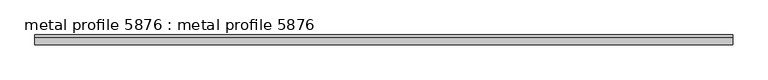
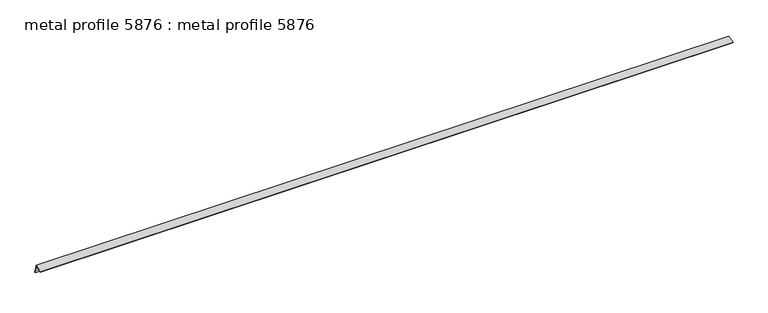
"""IFC4 building model written with IfcOpenShell, lengths in millimetres: proxy geometry, metal profile 5876 : metal profile 5876."""

import ifcopenshell
import ifcopenshell.guid

model = None  # the IFC model being written
_history = None  # IfcOwnerHistory: only IFC2X3 demands one
_inside = {}  # id of a spatial element -> (the spatial element, [elements in it])
_under = {}  # id of a project, library or spatial element -> (it, [spatial elements below it])
_declared = {}  # id of a project -> (the project, [libraries it declares])
_typed = {}  # id of a type object -> (the type object, [elements of that type])
_made_of = {}  # id of a material, layer set ... -> (it, [elements and type objects made of it])


def new_model(schema):
    """Start an empty IFC model of exactly this schema.

    Asked for "IFC4X3", IfcOpenShell would pick the latest addendum, in which some entities
    have other attributes; the version numbers below select the first issue.
    IFC2X3 requires an IfcOwnerHistory on every rooted entity: one is made here for all.
    """
    global model, _history
    if schema == "IFC4X3":
        model = ifcopenshell.file(schema_version=(4, 3, 0, 0))
    else:
        model = ifcopenshell.file(schema=schema)
    _inside.clear()
    _under.clear()
    _declared.clear()
    _typed.clear()
    _made_of.clear()
    _history = None
    if model.schema == "IFC2X3":
        org = make("IfcOrganization", Name="unknown")
        user = make(
            "IfcPersonAndOrganization",
            ThePerson=make("IfcPerson", FamilyName="unknown"),
            TheOrganization=org,
        )
        app = make(
            "IfcApplication",
            ApplicationDeveloper=org,
            Version="unknown",
            ApplicationFullName="unknown",
            ApplicationIdentifier="unknown",
        )
        _history = make(
            "IfcOwnerHistory",
            OwningUser=user,
            OwningApplication=app,
            ChangeAction="ADDED",
            CreationDate=0,
        )
    return model


def make(cls, **values):
    """One entity of the class cls with the attributes given. An attribute that is None is left unset."""
    return model.create_entity(
        cls, **{name: value for name, value in values.items() if value is not None}
    )


def rooted(cls, **values):
    """An entity with a GlobalId (a new one), such as an element, a storey or a relation."""
    return make(cls, GlobalId=ifcopenshell.guid.new(), OwnerHistory=_history, **values)


def si_unit(unit_type, name, prefix=None):
    """IfcSIUnit, for example si_unit("LENGTHUNIT", "METRE", prefix="MILLI")."""
    return make("IfcSIUnit", UnitType=unit_type, Prefix=prefix, Name=name)


def assignment(units):
    """IfcUnitAssignment: the units of a project."""
    return None if units is None else make("IfcUnitAssignment", Units=units)


def point(xyz):
    """IfcCartesianPoint."""
    return None if xyz is None else make("IfcCartesianPoint", Coordinates=xyz)


def direction(xyz):
    """IfcDirection."""
    return None if xyz is None else make("IfcDirection", DirectionRatios=xyz)


def frame(location, z_axis=None, x_axis=None):
    """IfcAxis2Placement3D, a coordinate frame: its origin and axes. An axis left out is left unset."""
    return make(
        "IfcAxis2Placement3D",
        Location=point(location),
        Axis=direction(z_axis),
        RefDirection=direction(x_axis),
    )


def origin():
    """The frame at (0, 0, 0) with its axes left unset."""
    return frame((0.0, 0.0, 0.0))


def place(relative_to, where):
    """IfcLocalPlacement: puts the frame where relative to a parent placement (None: the world)."""
    return make(
        "IfcLocalPlacement", PlacementRelTo=relative_to, RelativePlacement=where
    )


def context(
    kind, dimensions, precision=None, world=None, true_north=None, identifier=None
):
    """IfcGeometricRepresentationContext, for example the 3D "Model" context."""
    return make(
        "IfcGeometricRepresentationContext",
        ContextIdentifier=identifier,
        ContextType=kind,
        CoordinateSpaceDimension=dimensions,
        Precision=precision,
        WorldCoordinateSystem=world,
        TrueNorth=true_north,
    )


def project(units=None, contexts=None):
    """IfcProject with its units and contexts."""
    return rooted(
        "IfcProject",
        Name="project",
        RepresentationContexts=contexts,
        UnitsInContext=assignment(units),
    )


def spatial(cls, under=None, at=None, **own):
    """A site, building, storey or space (cls), placed at a placement, below another one or the project."""
    s = rooted(cls, ObjectPlacement=at, **own)
    if under is not None:
        _under.setdefault(under.id(), (under, []))[1].append(s)
    return s


def polyline(points):
    """IfcPolyline through the points."""
    return make("IfcPolyline", Points=[point(p) for p in points])


def outline(outer, holes=None, kind="AREA"):
    """IfcArbitraryClosedProfileDef: a profile drawn as a closed curve; with holes, ...WithVoids."""
    if holes is None:
        return make("IfcArbitraryClosedProfileDef", ProfileType=kind, OuterCurve=outer)
    return make(
        "IfcArbitraryProfileDefWithVoids",
        ProfileType=kind,
        OuterCurve=outer,
        InnerCurves=holes,
    )


def extrude(swept, where, along, depth):
    """IfcExtrudedAreaSolid: the profile swept, set in the frame where, extruded along a direction by depth."""
    return make(
        "IfcExtrudedAreaSolid",
        SweptArea=swept,
        Position=where,
        ExtrudedDirection=direction(along),
        Depth=depth,
    )


def shape(context_of_items, identifier, shape_type, items):
    """IfcShapeRepresentation: the items that make up one representation, for example the "Body"."""
    return make(
        "IfcShapeRepresentation",
        ContextOfItems=context_of_items,
        RepresentationIdentifier=identifier,
        RepresentationType=shape_type,
        Items=items,
    )


def source(mapping_origin, context_of_items, identifier, shape_type, items):
    """IfcRepresentationMap: a shape defined once, which mapped items show again and again."""
    return make(
        "IfcRepresentationMap",
        MappingOrigin=mapping_origin,
        MappedRepresentation=shape(context_of_items, identifier, shape_type, items),
    )


def transform(
    local_origin,
    x_axis=None,
    y_axis=None,
    z_axis=None,
    scale=None,
    scale2=None,
    scale3=None,
    uniform=True,
):
    """IfcCartesianTransformationOperator3D, or its non-uniform kind. x_axis, y_axis, z_axis: its Axis1, 2, 3."""
    if uniform:
        return make(
            "IfcCartesianTransformationOperator3D",
            Axis1=direction(x_axis),
            Axis2=direction(y_axis),
            LocalOrigin=point(local_origin),
            Scale=scale,
            Axis3=direction(z_axis),
        )
    return make(
        "IfcCartesianTransformationOperator3DnonUniform",
        Axis1=direction(x_axis),
        Axis2=direction(y_axis),
        LocalOrigin=point(local_origin),
        Scale=scale,
        Axis3=direction(z_axis),
        Scale2=scale2,
        Scale3=scale3,
    )


def mapped(mapping_source, mapping_target):
    """IfcMappedItem: shows the shape of a source again, moved by a transform."""
    return make(
        "IfcMappedItem", MappingSource=mapping_source, MappingTarget=mapping_target
    )


def made_of(thing, what):
    """Note that an element or type object is made of a material, layer set ...; save() writes the relation."""
    if what is not None:
        _made_of.setdefault(what.id(), (what, []))[1].append(thing)
    return thing


def element(
    cls,
    number,
    at=None,
    inside=None,
    cuts=None,
    type_object=None,
    material=None,
    context=None,
    identifier="Body",
    shape_type=None,
    held_by="IfcProductDefinitionShape",
    body=None,
    shapes=None,
    **own,
):
    """One element of the class cls, such as IfcWall. Its Tag is "e" and its number.

    at: its placement. inside: the storey or other place that contains it. cuts: it is an
    opening in that element (IfcRelVoidsElement). A single representation is given by context,
    identifier, shape_type and body (its items); several are given by shapes. held_by: the class
    of the entity that holds the representations. save() writes the other relations.
    """
    e = rooted(cls, Tag="e%d" % number, ObjectPlacement=at, **own)
    if body is not None:
        shapes = [shape(context, identifier, shape_type, body)]
    if shapes is not None:
        e.Representation = make(held_by, Representations=shapes)
    if inside is not None:
        _inside.setdefault(inside.id(), (inside, []))[1].append(e)
    if cuts is not None:
        rooted(
            "IfcRelVoidsElement", RelatingBuildingElement=cuts, RelatedOpeningElement=e
        )
    if type_object is not None:
        _typed.setdefault(type_object.id(), (type_object, []))[1].append(e)
    return made_of(e, material)


def aggregate(whole, parts):
    """IfcRelAggregates: a whole, such as a stair, and the parts it consists of."""
    return rooted("IfcRelAggregates", RelatingObject=whole, RelatedObjects=parts)


def save(model, path):
    """Write the relations noted so far, then the file.

    IfcRelAggregates (storeys below a building ...), IfcRelContainedInSpatialStructure (elements
    in a storey), IfcRelDefinesByType, IfcRelAssociatesMaterial and IfcRelDeclares: one each for
    every whole, place, type object, material and project.
    """
    for whole, parts in _under.values():
        aggregate(whole, parts)
    for where, things in _inside.values():
        rooted(
            "IfcRelContainedInSpatialStructure",
            RelatedElements=things,
            RelatingStructure=where,
        )
    for kind, things in _typed.values():
        rooted("IfcRelDefinesByType", RelatedObjects=things, RelatingType=kind)
    for what, things in _made_of.values():
        rooted("IfcRelAssociatesMaterial", RelatedObjects=things, RelatingMaterial=what)
    for by, libraries in _declared.values():
        rooted("IfcRelDeclares", RelatingContext=by, RelatedDefinitions=libraries)
    model.write(path)


def metal_profile_5876_metal_profile_5876_f78881de(model_context):
    return source(origin(), model_context, "Body", "SweptSolid", [
        extrude(outline(polyline([(-4228.2961988, 42682.9719046), (-4222.1357939, 42658.3302851), (-4224.0760789, 42657.8452139), (-4229.7539448, 42680.5566772), (-4249.4391531, 42675.7447028), (-4249.9140625, 42677.6875), (-4228.2961988, 42682.9719046)])), frame((12383.0178845, 0.0, 0.0), z_axis=(1.0, 0.0, 0.0), x_axis=(0.0, 1.0, 0.0)), (0.0, 0.0, 1.0), 2000.0),
    ])


if __name__ == "__main__":
    model = new_model("IFC4")
    model_context = context("Model", 3, world=origin())
    ifc_project = project(units=[si_unit("LENGTHUNIT", "METRE", prefix="MILLI")], contexts=[model_context])
    site = spatial("IfcSite", under=ifc_project)
    building = spatial("IfcBuilding", under=site)
    placement = place(None, origin())
    metal_profile_5876_metal_profile_5876_shape = metal_profile_5876_metal_profile_5876_f78881de(model_context)
    element("IfcBuildingElementProxy", 1, Name="metal profile 5876 : metal profile 5876", ObjectType="metal profile 5876 : metal profile 5876", at=placement, inside=building, context=model_context, shape_type="MappedRepresentation", body=[
        mapped(metal_profile_5876_metal_profile_5876_shape, transform((0.0, 0.0, 0.0), x_axis=(1.0, 0.0, 0.0), y_axis=(0.0, 1.0, 0.0), z_axis=(0.0, 0.0, 1.0))),
    ])
    save(model, "model.ifc")

# Revit data of these elements
# Type "metal profile 5876 : metal profile 5876"
#   NameOverride = "metal profile"
# Element 1 (IfcBuildingElementProxy, "metal profile 5876 : metal profile 5876")
#   Materials on its faces: "ANGLE TRIM 3448"
# Materials
#   "ANGLE TRIM 3448": class "Unassigned", colour RGB 234 229 0, transparency 0
